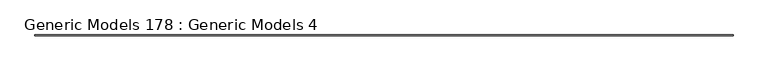
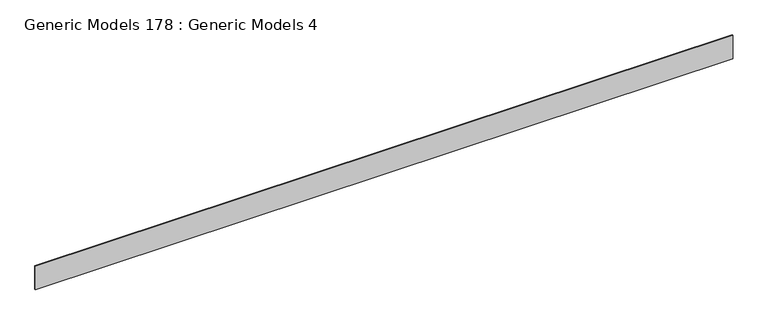
"""IFC4 building model written with IfcOpenShell, lengths in millimetres: proxy geometry, Generic Models 178 : Generic Models 4."""

from ifc_helpers import new_model, si_unit, frame, origin, place, context, project, spatial, polyline, outline, extrude, source, transform, mapped, element, save


def generic_models_178_generic_models_4_9fe66f18(model_context):
    return source(origin(), model_context, "Body", "SweptSolid", [
        extrude(outline(polyline([(0.0, -15.875), (0.0, 0.0), (12295.7684578, 0.0), (12295.7684578, -15.875), (0.0, -15.875)])), frame((2196.9263704, -5308.6625551, 126783.846), z_axis=(0.0, -1.0913936421275393e-12, 1.0), x_axis=(-1.0, 0.0, 0.0)), (0.0, 0.0, 1.0), 438.15),
    ])


if __name__ == "__main__":
    model = new_model("IFC4")
    model_context = context("Model", 3, world=origin())
    ifc_project = project(units=[si_unit("LENGTHUNIT", "METRE", prefix="MILLI")], contexts=[model_context])
    site = spatial("IfcSite", under=ifc_project)
    building = spatial("IfcBuilding", under=site)
    placement = place(None, origin())
    generic_models_178_generic_models_4_shape = generic_models_178_generic_models_4_9fe66f18(model_context)
    element("IfcBuildingElementProxy", 1, Name="Generic Models 178 : Generic Models 4", ObjectType="Generic Models 178 : Generic Models 4", at=placement, inside=building, context=model_context, shape_type="MappedRepresentation", body=[
        mapped(generic_models_178_generic_models_4_shape, transform((0.0, 0.0, 0.0), x_axis=(1.0, 0.0, 0.0), y_axis=(0.0, 1.0, 0.0), z_axis=(0.0, 0.0, 1.0))),
    ])
    save(model, "model.ifc")

# Revit data of these elements
# Element 1 (IfcBuildingElementProxy, "Generic Models 178 : Generic Models 4")
#   Materials on its faces: "_5/8\" DRYWALL"
# Materials
#   "_5/8\" DRYWALL": class "Generic", colour RGB 191 191 191, transparency 0, Cost = 0
